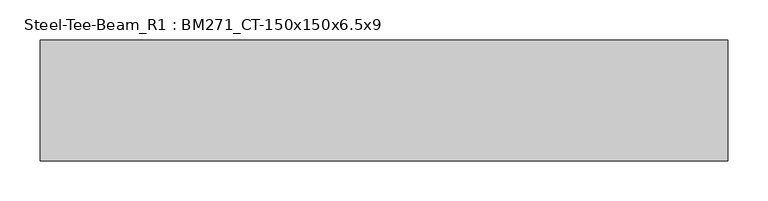
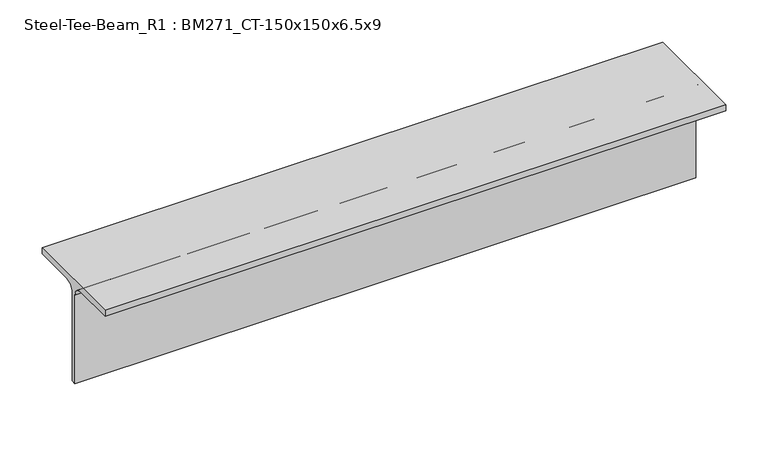
"""IFC4 building model written with IfcOpenShell, lengths in millimetres: member geometry, Steel-Tee-Beam_R1 : BM271_CT-150x150x6.5x9."""

from ifc_helpers import new_model, si_unit, point, frame, frame_2d, origin, place, context, project, spatial, polyline, circle_curve, trimmed, segment, composite_curve, outline, extrude, source, transform, mapped, element, save


def steel_tee_beam_r1_bm271_ct_150x150x6_5x9_cb24f347(model_context):
    return source(origin(), model_context, "Body", "SweptSolid", [
        extrude(outline(composite_curve([segment(polyline([(75.0, 75.0), (75.0, 66.0), (16.25, 66.0)]), True, "CONTINUOUS"), segment(trimmed(circle_curve(frame_2d((16.25, 53.0)), 13.0), [point((16.25, 66.0))], [point((3.25, 53.0))], True, "CARTESIAN"), True, "CONTINUOUS"), segment(polyline([(3.25, 53.0), (3.25, -75.0), (-3.25, -75.0), (-3.25, 53.0)]), True, "CONTINUOUS"), segment(trimmed(circle_curve(frame_2d((-16.25, 53.0)), 13.0), [point((-3.25, 53.0))], [point((-16.25, 66.0))], True, "CARTESIAN"), True, "CONTINUOUS"), segment(polyline([(-16.25, 66.0), (-75.0, 66.0), (-75.0, 75.0), (75.0, 75.0)]), True, "CONTINUOUS")], self_intersect=False)), frame((-500.0, 0.0, 0.0), z_axis=(1.0, 0.0, 0.0), x_axis=(0.0, 1.0, 0.0)), (0.0, 0.0, 1.0), 853.0826681),
    ])


if __name__ == "__main__":
    model = new_model("IFC4")
    model_context = context("Model", 3, world=origin())
    ifc_project = project(units=[si_unit("LENGTHUNIT", "METRE", prefix="MILLI")], contexts=[model_context])
    site = spatial("IfcSite", under=ifc_project)
    building = spatial("IfcBuilding", under=site)
    placement = place(None, origin())
    steel_tee_beam_r1_bm271_ct_150x150x6_5x9_shape = steel_tee_beam_r1_bm271_ct_150x150x6_5x9_cb24f347(model_context)
    element("IfcMember", 1, ObjectType="Steel-Tee-Beam_R1 : BM271_CT-150x150x6.5x9", at=placement, inside=building, context=model_context, shape_type="MappedRepresentation", body=[
        mapped(steel_tee_beam_r1_bm271_ct_150x150x6_5x9_shape, transform((0.0, 0.0, 0.0), x_axis=(1.0, 0.0, 0.0), y_axis=(0.0, 1.0, 0.0), z_axis=(0.0, 0.0, 1.0))),
    ])
    save(model, "model.ifc")

# Revit data of these elements
# Type "Steel-Tee-Beam_R1 : BM271_CT-150x150x6.5x9"
#   Keynote = "CT-150x150x6.5x9"
#   Surface Area = 0.588841 m²/m
#   Section Area = 23.3904 cm²
#   Mass per Unit Length = 18.3614 kg/m
#   Length [instance default] = 1.5240 m
#   bf = 0.1500 m
#   d = 0.1500 m
#   k = 0.0220 m
#   r = 0.0130 m
#   tf = 0.0090 m
#   tw = 0.0065 m
#   hec_material4 [instance default] = none
#   hec_material3 [instance default] = none
#   hec_material2 [instance default] = none
#   hec_material1 [instance default] = none
#   Structural Material [instance default] = Steel, 45-345
#   Assembly Code = ""
# Element 1 (IfcMember, "Steel-Tee-Beam_R1 : BM271_CT-150x150x6.5x9")
#   Structural Material = none
# Materials
#   "Steel, 45-345": class "Metal", colour RGB 189 187 185, transparency 0, Description = "Steel 345 MPa", Cost = 0
